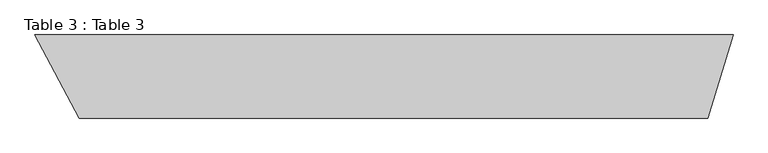
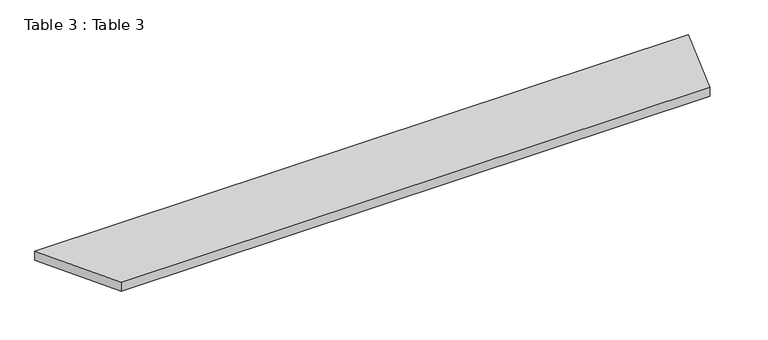
"""IFC4 building model written with IfcOpenShell, lengths in millimetres: furniture geometry, Table 3 : Table 3."""

from ifc_helpers import new_model, si_unit, point, frame, frame_2d, origin, place, context, project, spatial, polyline, circle_curve, trimmed, segment, composite_curve, outline, extrude, source, transform, mapped, element, save


def table_3_table_3_bbc5e5ae(model_context):
    return source(origin(), model_context, "Body", "SweptSolid", [
        extrude(outline(composite_curve([segment(trimmed(circle_curve(frame_2d((-6436.0739606, -13994.6059405)), 6213.6948928), [point((-11694.9835981, -17304.2696161))], [point((-12124.6753506, -16494.5696295))], False, "CARTESIAN"), True, "CONTINUOUS"), segment(polyline([(-12124.6753506, -16494.5696295), (-5323.914533, -16494.5696295)]), True, "CONTINUOUS"), segment(trimmed(circle_curve(frame_2d((-16626.7593666, -13519.9291403)), 11687.7195112), [point((-5323.914533, -16494.5696295))], [point((-5568.6603195, -17304.2696161))], False, "CARTESIAN"), True, "CONTINUOUS"), segment(polyline([(-5568.6603195, -17304.2696161), (-11694.9835981, -17304.2696161)]), True, "CONTINUOUS")], self_intersect=False)), frame((0.0, 0.0, 600.0), z_axis=(0.0, 0.0, 1.0), x_axis=(1.0, 0.0, 0.0)), (0.0, 0.0, 1.0), 100.0),
    ])


if __name__ == "__main__":
    model = new_model("IFC4")
    model_context = context("Model", 3, world=origin())
    ifc_project = project(units=[si_unit("LENGTHUNIT", "METRE", prefix="MILLI")], contexts=[model_context])
    site = spatial("IfcSite", under=ifc_project)
    building = spatial("IfcBuilding", under=site)
    placement = place(None, origin())
    table_3_table_3_shape = table_3_table_3_bbc5e5ae(model_context)
    element("IfcFurniture", 1, ObjectType="Table 3 : Table 3", at=placement, inside=building, context=model_context, shape_type="MappedRepresentation", body=[
        mapped(table_3_table_3_shape, transform((0.0, 0.0, 0.0), x_axis=(1.0, 0.0, 0.0), y_axis=(0.0, 1.0, 0.0), z_axis=(0.0, 0.0, 1.0))),
    ])
    save(model, "model.ifc")

# Revit data of these elements
# Type "Table 3 : Table 3"
#   COBie.Type.CreatedBy = "design@eagle.com"
#   COBie.Type.CreatedOn = "2016-09-13T05:47:35"
#   COBie.Type.Name = "Furniture_Table 3_Table 3"
#   COBie.Type.Category = "23-40 70 14 64 11 : Office Furniture"
#   COBie.Type.Description = ""
#   COBie.Type.Manufacturer = ""
#   COBie.Type.ModelNumber = ""
#   COBie.Type.ReplacementCost = 0
#   COBie.Type = yes
